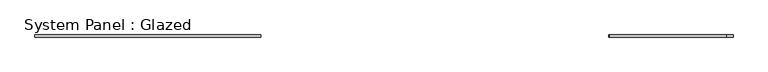
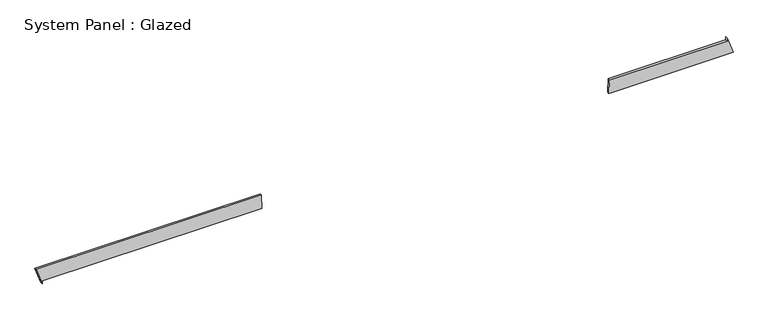
"""IFC4 building model written with IfcOpenShell, lengths in millimetres: plate geometry, System Panel : Glazed."""

from ifc_helpers import new_model, si_unit, frame, origin, place, context, project, spatial, polyline, outline, extrude, source, transform, mapped, element, save


def system_panel_glazed_22199b68(model_context):
    return source(origin(), model_context, "Body", "SweptSolid", [
        extrude(outline(polyline([(35.3553391, 2592.9093212), (35.3553391, 4027.1398136), (235.0472205, 3956.767991), (199.6918814, 3956.7680004), (199.6915206, 2596.4691848), (35.3553391, 2592.9093212)])), frame((0.0, -49.5, 0.0), z_axis=(0.0, 1.0, 0.0), x_axis=(0.0, 0.0, 1.0)), (0.0, 0.0, 1.0), 25.0),
        extrude(outline(polyline([(0.0, -3956.7629895), (35.3553391, -3956.7629895), (35.3553391, -1422.2011532), (199.6904543, -1424.1483538), (199.6897639, -4027.1398136), (0.0, -3956.7629895)])), frame((0.0, -49.5, 0.0), z_axis=(0.0, 1.0, 0.0), x_axis=(0.0, 0.0, 1.0)), (0.0, 0.0, 1.0), 25.0),
    ])


if __name__ == "__main__":
    model = new_model("IFC4")
    model_context = context("Model", 3, world=origin())
    ifc_project = project(units=[si_unit("LENGTHUNIT", "METRE", prefix="MILLI")], contexts=[model_context])
    site = spatial("IfcSite", under=ifc_project)
    building = spatial("IfcBuilding", under=site)
    placement = place(None, origin())
    system_panel_glazed_shape = system_panel_glazed_22199b68(model_context)
    element("IfcPlate", 1, ObjectType="System Panel : Glazed", at=placement, inside=building, context=model_context, shape_type="MappedRepresentation", body=[
        mapped(system_panel_glazed_shape, transform((0.0, 0.0, 0.0), x_axis=(1.0, 0.0, 0.0), y_axis=(0.0, 1.0, 0.0), z_axis=(0.0, 0.0, 1.0))),
    ])
    save(model, "model.ifc")

# Revit data of these elements
# Element 1 (IfcPlate, "System Panel : Glazed")
#   Materials on its faces: "Glass"
# Materials
#   "Glass": class "Glass", colour RGB 218 227 224, transparency 0.85, Description = "Soda Lime Glass", Cost = 0
